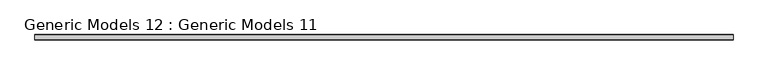
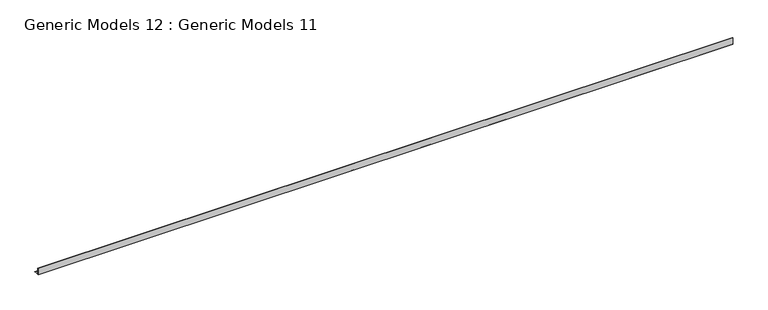
"""IFC4 building model written with IfcOpenShell, lengths in millimetres: proxy geometry, Generic Models 12 : Generic Models 11."""

from ifc_helpers import new_model, si_unit, frame, origin, place, context, project, spatial, polyline, outline, extrude, source, transform, mapped, element, save


def generic_models_12_generic_models_11_016286e5(model_context):
    return source(origin(), model_context, "Body", "SweptSolid", [
        extrude(outline(polyline([(40957.8387657, 269343.3815726), (40957.8387657, 269398.9440726), (40959.4262657, 269398.9440726), (40959.4262657, 269344.9690726), (40997.8407891, 269344.9690726), (41002.3309171, 269340.4789445), (41001.2083851, 269339.3564125), (40997.183225, 269343.3815726), (40957.8387657, 269343.3815726)])), frame((26424.3233872, 0.0, 0.0), z_axis=(1.0, 0.0, 0.0), x_axis=(0.0, 1.0, 0.0)), (0.0, 0.0, 1.0), 5752.7106906),
    ])


if __name__ == "__main__":
    model = new_model("IFC4")
    model_context = context("Model", 3, world=origin())
    ifc_project = project(units=[si_unit("LENGTHUNIT", "METRE", prefix="MILLI")], contexts=[model_context])
    site = spatial("IfcSite", under=ifc_project)
    building = spatial("IfcBuilding", under=site)
    placement = place(None, origin())
    generic_models_12_generic_models_11_shape = generic_models_12_generic_models_11_016286e5(model_context)
    element("IfcBuildingElementProxy", 1, Name="Generic Models 12 : Generic Models 11", ObjectType="Generic Models 12 : Generic Models 11", at=placement, inside=building, context=model_context, shape_type="MappedRepresentation", body=[
        mapped(generic_models_12_generic_models_11_shape, transform((0.0, 0.0, 0.0), x_axis=(1.0, 0.0, 0.0), y_axis=(0.0, 1.0, 0.0), z_axis=(0.0, 0.0, 1.0))),
    ])
    save(model, "model.ifc")

# Revit data of these elements
# Project information
#   Project Issue Date = "02.05.2018"
#   Project Status = "Project Status"
#   Client Name = "Owner"
#   Project Address = "640 West Main Street, Lake Geneva, WI 53147"
#   Project Name = "The Downtowner"
#   Project Number = "Project Number"
# Element 1 (IfcBuildingElementProxy, "Generic Models 12 : Generic Models 11")
#   Materials on its faces: "GALV. BRAKE METAL - (COLOR: GALV.)"
# Materials
#   "GALV. BRAKE METAL - (COLOR: GALV.)": class "Generic", colour RGB 234 234 234, transparency 0, Cost = 0
